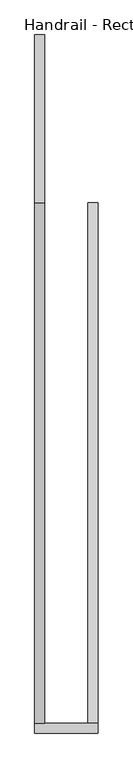
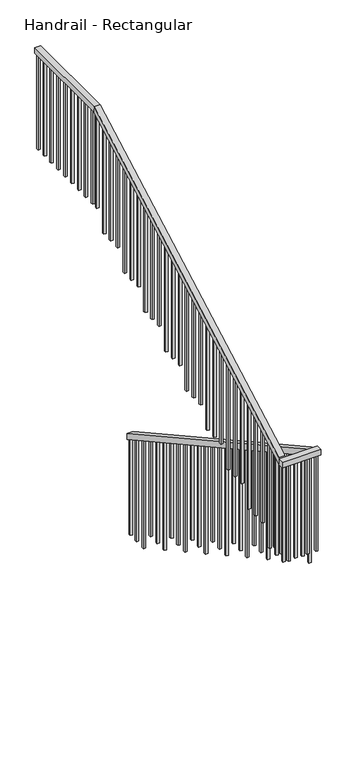
"""IFC4 building model written with IfcOpenShell, lengths in millimetres: railing geometry, Handrail - Rectangular."""

from ifc_helpers import new_model, si_unit, frame, origin, place, context, project, spatial, polyline, outline, extrude, faceted_brep, source, transform, mapped, element, save


def handrail_rectangular_766db315(model_context):
    return source(origin(), model_context, "Body", "SolidModel", [
        faceted_brep([(-74723.577375, 13792.2, 13481.05), (-74723.577375, 13792.2, 13430.25), (-74774.377375, 13792.2, 13430.25), (-74774.377375, 13792.2, 13481.05), (-74723.577375, 12915.9, 13481.05), (-74723.577375, 12929.0029811, 13430.25), (-74774.377375, 12929.0029811, 13430.25), (-74774.377375, 12915.9, 13481.05), (-74723.577375, 10198.1, 11979.1078947), (-74774.377375, 10198.1, 11979.1078947), (-74774.377375, 10198.1, 11921.0667736), (-74723.577375, 10198.1, 11921.0667736)], [[[0, 1, 2, 3]], [[1, 0, 4, 5]], [[2, 1, 5, 6]], [[3, 2, 6, 7]], [[0, 3, 7, 4]], [[8, 9, 10, 11]], [[5, 4, 8, 11]], [[6, 5, 11, 10]], [[7, 6, 10, 9]], [[4, 7, 9, 8]]]),
        faceted_brep([(-74774.377375, 10198.1, 11965.0710526), (-74774.377375, 10198.1, 11914.2710526), (-74774.377375, 10147.3, 11914.2710526), (-74774.377375, 10147.3, 11965.0710526), (-74444.177375, 10198.1, 11965.0710526), (-74444.177375, 10147.3, 11965.0710526), (-74444.177375, 10147.3, 11914.2710526), (-74444.177375, 10198.1, 11914.2710526)], [[[0, 1, 2, 3]], [[4, 5, 6, 7]], [[1, 0, 4, 7]], [[2, 1, 7, 6]], [[3, 2, 6, 5]], [[0, 3, 5, 4]]]),
        faceted_brep([(-74494.977375, 10198.1, 11951.0342105), (-74494.977375, 10198.1, 11892.9930894), (-74444.177375, 10198.1, 11892.9930894), (-74444.177375, 10198.1, 11951.0342105), (-74494.977375, 12915.9, 10449.0921053), (-74444.177375, 12915.9, 10449.0921053), (-74444.177375, 12915.9, 10391.0509841), (-74494.977375, 12915.9, 10391.0509841)], [[[0, 1, 2, 3]], [[4, 5, 6, 7]], [[1, 0, 4, 7]], [[2, 1, 7, 6]], [[3, 2, 6, 5]], [[0, 3, 5, 4]]]),
        extrude(outline(polyline([(12823.825, 10441.9345367), (12823.825, 9534.6921053), (12804.775, 9534.6921053), (12804.775, 10452.4621683), (12823.825, 10441.9345367)])), frame((-74479.102375, 0.0, 0.0), z_axis=(1.0, 0.0, 0.0), x_axis=(0.0, 1.0, 0.0)), (0.0, 0.0, 1.0), 19.05),
        extrude(outline(polyline([(12722.225, 10498.0819052), (12722.225, 9534.6921053), (12703.175, 9534.6921053), (12703.175, 10508.6095367), (12722.225, 10498.0819052)])), frame((-74479.102375, 0.0, 0.0), z_axis=(1.0, 0.0, 0.0), x_axis=(0.0, 1.0, 0.0)), (0.0, 0.0, 1.0), 19.05),
        extrude(outline(polyline([(12620.625, 10554.2292736), (12620.625, 9703.1342105), (12601.575, 9703.1342105), (12601.575, 10564.7569052), (12620.625, 10554.2292736)])), frame((-74479.102375, 0.0, 0.0), z_axis=(1.0, 0.0, 0.0), x_axis=(0.0, 1.0, 0.0)), (0.0, 0.0, 1.0), 19.05),
        extrude(outline(polyline([(12519.025, 10610.376642), (12519.025, 9703.1342105), (12499.975, 9703.1342105), (12499.975, 10620.9042736), (12519.025, 10610.376642)])), frame((-74479.102375, 0.0, 0.0), z_axis=(1.0, 0.0, 0.0), x_axis=(0.0, 1.0, 0.0)), (0.0, 0.0, 1.0), 19.05),
        extrude(outline(polyline([(12417.425, 10666.5240104), (12417.425, 9703.1342105), (12398.375, 9703.1342105), (12398.375, 10677.051642), (12417.425, 10666.5240104)])), frame((-74479.102375, 0.0, 0.0), z_axis=(1.0, 0.0, 0.0), x_axis=(0.0, 1.0, 0.0)), (0.0, 0.0, 1.0), 19.05),
        extrude(outline(polyline([(12315.825, 10722.6713788), (12315.825, 9871.5763158), (12296.775, 9871.5763158), (12296.775, 10733.1990104), (12315.825, 10722.6713788)])), frame((-74479.102375, 0.0, 0.0), z_axis=(1.0, 0.0, 0.0), x_axis=(0.0, 1.0, 0.0)), (0.0, 0.0, 1.0), 19.05),
        extrude(outline(polyline([(12214.225, 10778.8187473), (12214.225, 9871.5763158), (12195.175, 9871.5763158), (12195.175, 10789.3463788), (12214.225, 10778.8187473)])), frame((-74479.102375, 0.0, 0.0), z_axis=(1.0, 0.0, 0.0), x_axis=(0.0, 1.0, 0.0)), (0.0, 0.0, 1.0), 19.05),
        extrude(outline(polyline([(12112.625, 10834.9661157), (12112.625, 9871.5763158), (12093.575, 9871.5763158), (12093.575, 10845.4937473), (12112.625, 10834.9661157)])), frame((-74479.102375, 0.0, 0.0), z_axis=(1.0, 0.0, 0.0), x_axis=(0.0, 1.0, 0.0)), (0.0, 0.0, 1.0), 19.05),
        extrude(outline(polyline([(12011.025, 10891.1134841), (12011.025, 10040.0184211), (11991.975, 10040.0184211), (11991.975, 10901.6411157), (12011.025, 10891.1134841)])), frame((-74479.102375, 0.0, 0.0), z_axis=(1.0, 0.0, 0.0), x_axis=(0.0, 1.0, 0.0)), (0.0, 0.0, 1.0), 19.05),
        extrude(outline(polyline([(11909.425, 10947.2608525), (11909.425, 10040.0184211), (11890.375, 10040.0184211), (11890.375, 10957.7884841), (11909.425, 10947.2608525)])), frame((-74479.102375, 0.0, 0.0), z_axis=(1.0, 0.0, 0.0), x_axis=(0.0, 1.0, 0.0)), (0.0, 0.0, 1.0), 19.05),
        extrude(outline(polyline([(11807.825, 11003.4082209), (11807.825, 10040.0184211), (11788.775, 10040.0184211), (11788.775, 11013.9358525), (11807.825, 11003.4082209)])), frame((-74479.102375, 0.0, 0.0), z_axis=(1.0, 0.0, 0.0), x_axis=(0.0, 1.0, 0.0)), (0.0, 0.0, 1.0), 19.05),
        extrude(outline(polyline([(11706.225, 11059.5555894), (11706.225, 10208.4605263), (11687.175, 10208.4605263), (11687.175, 11070.0832209), (11706.225, 11059.5555894)])), frame((-74479.102375, 0.0, 0.0), z_axis=(1.0, 0.0, 0.0), x_axis=(0.0, 1.0, 0.0)), (0.0, 0.0, 1.0), 19.05),
        extrude(outline(polyline([(11604.625, 11115.7029578), (11604.625, 10208.4605263), (11585.575, 10208.4605263), (11585.575, 11126.2305894), (11604.625, 11115.7029578)])), frame((-74479.102375, 0.0, 0.0), z_axis=(1.0, 0.0, 0.0), x_axis=(0.0, 1.0, 0.0)), (0.0, 0.0, 1.0), 19.05),
        extrude(outline(polyline([(11503.025, 11171.8503262), (11503.025, 10208.4605263), (11483.975, 10208.4605263), (11483.975, 11182.3779578), (11503.025, 11171.8503262)])), frame((-74479.102375, 0.0, 0.0), z_axis=(1.0, 0.0, 0.0), x_axis=(0.0, 1.0, 0.0)), (0.0, 0.0, 1.0), 19.05),
        extrude(outline(polyline([(11401.425, 11227.9976946), (11401.425, 10376.9026316), (11382.375, 10376.9026316), (11382.375, 11238.5253262), (11401.425, 11227.9976946)])), frame((-74479.102375, 0.0, 0.0), z_axis=(1.0, 0.0, 0.0), x_axis=(0.0, 1.0, 0.0)), (0.0, 0.0, 1.0), 19.05),
        extrude(outline(polyline([(11299.825, 11284.1450631), (11299.825, 10376.9026316), (11280.775, 10376.9026316), (11280.775, 11294.6726946), (11299.825, 11284.1450631)])), frame((-74479.102375, 0.0, 0.0), z_axis=(1.0, 0.0, 0.0), x_axis=(0.0, 1.0, 0.0)), (0.0, 0.0, 1.0), 19.05),
        extrude(outline(polyline([(11198.225, 11340.2924315), (11198.225, 10376.9026316), (11179.175, 10376.9026316), (11179.175, 11350.8200631), (11198.225, 11340.2924315)])), frame((-74479.102375, 0.0, 0.0), z_axis=(1.0, 0.0, 0.0), x_axis=(0.0, 1.0, 0.0)), (0.0, 0.0, 1.0), 19.05),
        extrude(outline(polyline([(11096.625, 11396.4397999), (11096.625, 10545.3447368), (11077.575, 10545.3447368), (11077.575, 11406.9674315), (11096.625, 11396.4397999)])), frame((-74479.102375, 0.0, 0.0), z_axis=(1.0, 0.0, 0.0), x_axis=(0.0, 1.0, 0.0)), (0.0, 0.0, 1.0), 19.05),
        extrude(outline(polyline([(10995.025, 11452.5871683), (10995.025, 10545.3447368), (10975.975, 10545.3447368), (10975.975, 11463.1147999), (10995.025, 11452.5871683)])), frame((-74479.102375, 0.0, 0.0), z_axis=(1.0, 0.0, 0.0), x_axis=(0.0, 1.0, 0.0)), (0.0, 0.0, 1.0), 19.05),
        extrude(outline(polyline([(10893.425, 11508.7345367), (10893.425, 10545.3447368), (10874.375, 10545.3447368), (10874.375, 11519.2621683), (10893.425, 11508.7345367)])), frame((-74479.102375, 0.0, 0.0), z_axis=(1.0, 0.0, 0.0), x_axis=(0.0, 1.0, 0.0)), (0.0, 0.0, 1.0), 19.05),
        extrude(outline(polyline([(10791.825, 11564.8819052), (10791.825, 10713.7868421), (10772.775, 10713.7868421), (10772.775, 11575.4095367), (10791.825, 11564.8819052)])), frame((-74479.102375, 0.0, 0.0), z_axis=(1.0, 0.0, 0.0), x_axis=(0.0, 1.0, 0.0)), (0.0, 0.0, 1.0), 19.05),
        extrude(outline(polyline([(10690.225, 11621.0292736), (10690.225, 10713.7868421), (10671.175, 10713.7868421), (10671.175, 11631.5569052), (10690.225, 11621.0292736)])), frame((-74479.102375, 0.0, 0.0), z_axis=(1.0, 0.0, 0.0), x_axis=(0.0, 1.0, 0.0)), (0.0, 0.0, 1.0), 19.05),
        extrude(outline(polyline([(10588.625, 11677.176642), (10588.625, 10713.7868421), (10569.575, 10713.7868421), (10569.575, 11687.7042736), (10588.625, 11677.176642)])), frame((-74479.102375, 0.0, 0.0), z_axis=(1.0, 0.0, 0.0), x_axis=(0.0, 1.0, 0.0)), (0.0, 0.0, 1.0), 19.05),
        extrude(outline(polyline([(10487.025, 11733.3240104), (10487.025, 10882.2289474), (10467.975, 10882.2289474), (10467.975, 11743.851642), (10487.025, 11733.3240104)])), frame((-74479.102375, 0.0, 0.0), z_axis=(1.0, 0.0, 0.0), x_axis=(0.0, 1.0, 0.0)), (0.0, 0.0, 1.0), 19.05),
        extrude(outline(polyline([(10385.425, 11789.4713788), (10385.425, 10882.2289474), (10366.375, 10882.2289474), (10366.375, 11799.9990104), (10385.425, 11789.4713788)])), frame((-74479.102375, 0.0, 0.0), z_axis=(1.0, 0.0, 0.0), x_axis=(0.0, 1.0, 0.0)), (0.0, 0.0, 1.0), 19.05),
        extrude(outline(polyline([(10283.825, 11845.6187473), (10283.825, 10882.2289474), (10264.775, 10882.2289474), (10264.775, 11856.1463788), (10283.825, 11845.6187473)])), frame((-74479.102375, 0.0, 0.0), z_axis=(1.0, 0.0, 0.0), x_axis=(0.0, 1.0, 0.0)), (0.0, 0.0, 1.0), 19.05),
        extrude(outline(polyline([(-74555.302375, 10182.225), (-74536.252375, 10182.225), (-74536.252375, 10163.175), (-74555.302375, 10163.175), (-74555.302375, 10182.225)])), frame((0.0, 0.0, 11050.6710526), z_axis=(0.0, 0.0, 1.0), x_axis=(1.0, 0.0, 0.0)), (0.0, 0.0, 1.0), 863.6),
        extrude(outline(polyline([(-74656.902375, 10182.225), (-74637.852375, 10182.225), (-74637.852375, 10163.175), (-74656.902375, 10163.175), (-74656.902375, 10182.225)])), frame((0.0, 0.0, 11050.6710526), z_axis=(0.0, 0.0, 1.0), x_axis=(1.0, 0.0, 0.0)), (0.0, 0.0, 1.0), 863.6),
        extrude(outline(polyline([(10283.825, 11968.4411157), (10283.825, 11050.6710526), (10264.775, 11050.6710526), (10264.775, 11957.9134841), (10283.825, 11968.4411157)])), frame((-74758.502375, 0.0, 0.0), z_axis=(1.0, 0.0, 0.0), x_axis=(0.0, 1.0, 0.0)), (0.0, 0.0, 1.0), 19.05),
        extrude(outline(polyline([(10385.425, 12024.5884841), (10385.425, 11050.6710526), (10366.375, 11050.6710526), (10366.375, 12014.0608525), (10385.425, 12024.5884841)])), frame((-74758.502375, 0.0, 0.0), z_axis=(1.0, 0.0, 0.0), x_axis=(0.0, 1.0, 0.0)), (0.0, 0.0, 1.0), 19.05),
        extrude(outline(polyline([(10487.025, 12080.7358525), (10487.025, 11219.1131579), (10467.975, 11219.1131579), (10467.975, 12070.2082209), (10487.025, 12080.7358525)])), frame((-74758.502375, 0.0, 0.0), z_axis=(1.0, 0.0, 0.0), x_axis=(0.0, 1.0, 0.0)), (0.0, 0.0, 1.0), 19.05),
        extrude(outline(polyline([(10588.625, 12136.8832209), (10588.625, 11219.1131579), (10569.575, 11219.1131579), (10569.575, 12126.3555894), (10588.625, 12136.8832209)])), frame((-74758.502375, 0.0, 0.0), z_axis=(1.0, 0.0, 0.0), x_axis=(0.0, 1.0, 0.0)), (0.0, 0.0, 1.0), 19.05),
        extrude(outline(polyline([(10690.225, 12193.0305894), (10690.225, 11219.1131579), (10671.175, 11219.1131579), (10671.175, 12182.5029578), (10690.225, 12193.0305894)])), frame((-74758.502375, 0.0, 0.0), z_axis=(1.0, 0.0, 0.0), x_axis=(0.0, 1.0, 0.0)), (0.0, 0.0, 1.0), 19.05),
        extrude(outline(polyline([(10791.825, 12249.1779578), (10791.825, 11387.5552632), (10772.775, 11387.5552632), (10772.775, 12238.6503262), (10791.825, 12249.1779578)])), frame((-74758.502375, 0.0, 0.0), z_axis=(1.0, 0.0, 0.0), x_axis=(0.0, 1.0, 0.0)), (0.0, 0.0, 1.0), 19.05),
        extrude(outline(polyline([(10893.425, 12305.3253262), (10893.425, 11387.5552632), (10874.375, 11387.5552632), (10874.375, 12294.7976946), (10893.425, 12305.3253262)])), frame((-74758.502375, 0.0, 0.0), z_axis=(1.0, 0.0, 0.0), x_axis=(0.0, 1.0, 0.0)), (0.0, 0.0, 1.0), 19.05),
        extrude(outline(polyline([(10995.025, 12361.4726946), (10995.025, 11387.5552632), (10975.975, 11387.5552632), (10975.975, 12350.9450631), (10995.025, 12361.4726946)])), frame((-74758.502375, 0.0, 0.0), z_axis=(1.0, 0.0, 0.0), x_axis=(0.0, 1.0, 0.0)), (0.0, 0.0, 1.0), 19.05),
        extrude(outline(polyline([(11096.625, 12417.6200631), (11096.625, 11555.9973684), (11077.575, 11555.9973684), (11077.575, 12407.0924315), (11096.625, 12417.6200631)])), frame((-74758.502375, 0.0, 0.0), z_axis=(1.0, 0.0, 0.0), x_axis=(0.0, 1.0, 0.0)), (0.0, 0.0, 1.0), 19.05),
        extrude(outline(polyline([(11198.225, 12473.7674315), (11198.225, 11555.9973684), (11179.175, 11555.9973684), (11179.175, 12463.2397999), (11198.225, 12473.7674315)])), frame((-74758.502375, 0.0, 0.0), z_axis=(1.0, 0.0, 0.0), x_axis=(0.0, 1.0, 0.0)), (0.0, 0.0, 1.0), 19.05),
        extrude(outline(polyline([(11299.825, 12529.9147999), (11299.825, 11555.9973684), (11280.775, 11555.9973684), (11280.775, 12519.3871683), (11299.825, 12529.9147999)])), frame((-74758.502375, 0.0, 0.0), z_axis=(1.0, 0.0, 0.0), x_axis=(0.0, 1.0, 0.0)), (0.0, 0.0, 1.0), 19.05),
        extrude(outline(polyline([(11401.425, 12586.0621683), (11401.425, 11724.4394737), (11382.375, 11724.4394737), (11382.375, 12575.5345367), (11401.425, 12586.0621683)])), frame((-74758.502375, 0.0, 0.0), z_axis=(1.0, 0.0, 0.0), x_axis=(0.0, 1.0, 0.0)), (0.0, 0.0, 1.0), 19.05),
        extrude(outline(polyline([(11503.025, 12642.2095367), (11503.025, 11724.4394737), (11483.975, 11724.4394737), (11483.975, 12631.6819052), (11503.025, 12642.2095367)])), frame((-74758.502375, 0.0, 0.0), z_axis=(1.0, 0.0, 0.0), x_axis=(0.0, 1.0, 0.0)), (0.0, 0.0, 1.0), 19.05),
        extrude(outline(polyline([(11604.625, 12698.3569052), (11604.625, 11724.4394737), (11585.575, 11724.4394737), (11585.575, 12687.8292736), (11604.625, 12698.3569052)])), frame((-74758.502375, 0.0, 0.0), z_axis=(1.0, 0.0, 0.0), x_axis=(0.0, 1.0, 0.0)), (0.0, 0.0, 1.0), 19.05),
        extrude(outline(polyline([(11706.225, 12754.5042736), (11706.225, 11892.8815789), (11687.175, 11892.8815789), (11687.175, 12743.976642), (11706.225, 12754.5042736)])), frame((-74758.502375, 0.0, 0.0), z_axis=(1.0, 0.0, 0.0), x_axis=(0.0, 1.0, 0.0)), (0.0, 0.0, 1.0), 19.05),
        extrude(outline(polyline([(11807.825, 12810.651642), (11807.825, 11892.8815789), (11788.775, 11892.8815789), (11788.775, 12800.1240104), (11807.825, 12810.651642)])), frame((-74758.502375, 0.0, 0.0), z_axis=(1.0, 0.0, 0.0), x_axis=(0.0, 1.0, 0.0)), (0.0, 0.0, 1.0), 19.05),
        extrude(outline(polyline([(11909.425, 12866.7990104), (11909.425, 11892.8815789), (11890.375, 11892.8815789), (11890.375, 12856.2713788), (11909.425, 12866.7990104)])), frame((-74758.502375, 0.0, 0.0), z_axis=(1.0, 0.0, 0.0), x_axis=(0.0, 1.0, 0.0)), (0.0, 0.0, 1.0), 19.05),
        extrude(outline(polyline([(12011.025, 12922.9463788), (12011.025, 12061.3236842), (11991.975, 12061.3236842), (11991.975, 12912.4187473), (12011.025, 12922.9463788)])), frame((-74758.502375, 0.0, 0.0), z_axis=(1.0, 0.0, 0.0), x_axis=(0.0, 1.0, 0.0)), (0.0, 0.0, 1.0), 19.05),
        extrude(outline(polyline([(12112.625, 12979.0937473), (12112.625, 12061.3236842), (12093.575, 12061.3236842), (12093.575, 12968.5661157), (12112.625, 12979.0937473)])), frame((-74758.502375, 0.0, 0.0), z_axis=(1.0, 0.0, 0.0), x_axis=(0.0, 1.0, 0.0)), (0.0, 0.0, 1.0), 19.05),
        extrude(outline(polyline([(12214.225, 13035.2411157), (12214.225, 12061.3236842), (12195.175, 12061.3236842), (12195.175, 13024.7134841), (12214.225, 13035.2411157)])), frame((-74758.502375, 0.0, 0.0), z_axis=(1.0, 0.0, 0.0), x_axis=(0.0, 1.0, 0.0)), (0.0, 0.0, 1.0), 19.05),
        extrude(outline(polyline([(12315.825, 13091.3884841), (12315.825, 12229.7657895), (12296.775, 12229.7657895), (12296.775, 13080.8608525), (12315.825, 13091.3884841)])), frame((-74758.502375, 0.0, 0.0), z_axis=(1.0, 0.0, 0.0), x_axis=(0.0, 1.0, 0.0)), (0.0, 0.0, 1.0), 19.05),
        extrude(outline(polyline([(12417.425, 13147.5358525), (12417.425, 12229.7657895), (12398.375, 12229.7657895), (12398.375, 13137.0082209), (12417.425, 13147.5358525)])), frame((-74758.502375, 0.0, 0.0), z_axis=(1.0, 0.0, 0.0), x_axis=(0.0, 1.0, 0.0)), (0.0, 0.0, 1.0), 19.05),
        extrude(outline(polyline([(12519.025, 13203.6832209), (12519.025, 12229.7657895), (12499.975, 12229.7657895), (12499.975, 13193.1555894), (12519.025, 13203.6832209)])), frame((-74758.502375, 0.0, 0.0), z_axis=(1.0, 0.0, 0.0), x_axis=(0.0, 1.0, 0.0)), (0.0, 0.0, 1.0), 19.05),
        extrude(outline(polyline([(12620.625, 13259.8305894), (12620.625, 12398.2078947), (12601.575, 12398.2078947), (12601.575, 13249.3029578), (12620.625, 13259.8305894)])), frame((-74758.502375, 0.0, 0.0), z_axis=(1.0, 0.0, 0.0), x_axis=(0.0, 1.0, 0.0)), (0.0, 0.0, 1.0), 19.05),
        extrude(outline(polyline([(12722.225, 13315.9779578), (12722.225, 12398.2078947), (12703.175, 12398.2078947), (12703.175, 13305.4503262), (12722.225, 13315.9779578)])), frame((-74758.502375, 0.0, 0.0), z_axis=(1.0, 0.0, 0.0), x_axis=(0.0, 1.0, 0.0)), (0.0, 0.0, 1.0), 19.05),
        extrude(outline(polyline([(12823.825, 13372.1253262), (12823.825, 12398.2078947), (12804.775, 12398.2078947), (12804.775, 13361.5976946), (12823.825, 13372.1253262)])), frame((-74758.502375, 0.0, 0.0), z_axis=(1.0, 0.0, 0.0), x_axis=(0.0, 1.0, 0.0)), (0.0, 0.0, 1.0), 19.05),
        extrude(outline(polyline([(-74739.452375, 12988.925), (-74739.452375, 12969.875), (-74758.502375, 12969.875), (-74758.502375, 12988.925), (-74739.452375, 12988.925)])), frame((0.0, 0.0, 12566.65), z_axis=(0.0, 0.0, 1.0), x_axis=(1.0, 0.0, 0.0)), (0.0, 0.0, 1.0), 863.6),
        extrude(outline(polyline([(-74739.452375, 13090.525), (-74739.452375, 13071.475), (-74758.502375, 13071.475), (-74758.502375, 13090.525), (-74739.452375, 13090.525)])), frame((0.0, 0.0, 12566.65), z_axis=(0.0, 0.0, 1.0), x_axis=(1.0, 0.0, 0.0)), (0.0, 0.0, 1.0), 863.6),
        extrude(outline(polyline([(-74739.452375, 13192.125), (-74739.452375, 13173.075), (-74758.502375, 13173.075), (-74758.502375, 13192.125), (-74739.452375, 13192.125)])), frame((0.0, 0.0, 12566.65), z_axis=(0.0, 0.0, 1.0), x_axis=(1.0, 0.0, 0.0)), (0.0, 0.0, 1.0), 863.6),
        extrude(outline(polyline([(-74739.452375, 13293.725), (-74739.452375, 13274.675), (-74758.502375, 13274.675), (-74758.502375, 13293.725), (-74739.452375, 13293.725)])), frame((0.0, 0.0, 12566.65), z_axis=(0.0, 0.0, 1.0), x_axis=(1.0, 0.0, 0.0)), (0.0, 0.0, 1.0), 863.6),
        extrude(outline(polyline([(-74739.452375, 13395.325), (-74739.452375, 13376.275), (-74758.502375, 13376.275), (-74758.502375, 13395.325), (-74739.452375, 13395.325)])), frame((0.0, 0.0, 12566.65), z_axis=(0.0, 0.0, 1.0), x_axis=(1.0, 0.0, 0.0)), (0.0, 0.0, 1.0), 863.6),
        extrude(outline(polyline([(-74739.452375, 13496.925), (-74739.452375, 13477.875), (-74758.502375, 13477.875), (-74758.502375, 13496.925), (-74739.452375, 13496.925)])), frame((0.0, 0.0, 12566.65), z_axis=(0.0, 0.0, 1.0), x_axis=(1.0, 0.0, 0.0)), (0.0, 0.0, 1.0), 863.6),
        extrude(outline(polyline([(-74739.452375, 13598.525), (-74739.452375, 13579.475), (-74758.502375, 13579.475), (-74758.502375, 13598.525), (-74739.452375, 13598.525)])), frame((0.0, 0.0, 12566.65), z_axis=(0.0, 0.0, 1.0), x_axis=(1.0, 0.0, 0.0)), (0.0, 0.0, 1.0), 863.6),
        extrude(outline(polyline([(-74739.452375, 13700.125), (-74739.452375, 13681.075), (-74758.502375, 13681.075), (-74758.502375, 13700.125), (-74739.452375, 13700.125)])), frame((0.0, 0.0, 12566.65), z_axis=(0.0, 0.0, 1.0), x_axis=(1.0, 0.0, 0.0)), (0.0, 0.0, 1.0), 863.6),
        extrude(outline(polyline([(-74479.102375, 10182.225), (-74460.052375, 10182.225), (-74460.052375, 10163.175), (-74479.102375, 10163.175), (-74479.102375, 10182.225)])), frame((0.0, 0.0, 11050.6710526), z_axis=(0.0, 0.0, 1.0), x_axis=(1.0, 0.0, 0.0)), (0.0, 0.0, 1.0), 863.6),
        extrude(outline(polyline([(10182.225, 11912.2937473), (10182.225, 11050.6710526), (10163.175, 11050.6710526), (10163.175, 11901.7661157), (10182.225, 11912.2937473)])), frame((-74758.502375, 0.0, 0.0), z_axis=(1.0, 0.0, 0.0), x_axis=(0.0, 1.0, 0.0)), (0.0, 0.0, 1.0), 19.05),
        extrude(outline(polyline([(-74739.452375, 12925.425), (-74739.452375, 12906.375), (-74758.502375, 12906.375), (-74758.502375, 12925.425), (-74739.452375, 12925.425)])), frame((0.0, 0.0, 12566.65), z_axis=(0.0, 0.0, 1.0), x_axis=(1.0, 0.0, 0.0)), (0.0, 0.0, 1.0), 863.6),
        extrude(outline(polyline([(12915.9, 10391.0509841), (12915.9, 9534.6921053), (12896.85, 9534.6921053), (12896.85, 10401.5786157), (12915.9, 10391.0509841)])), frame((-74479.102375, 0.0, 0.0), z_axis=(1.0, 0.0, 0.0), x_axis=(0.0, 1.0, 0.0)), (0.0, 0.0, 1.0), 19.05),
        extrude(outline(polyline([(-74739.452375, 13792.2), (-74739.452375, 13773.15), (-74758.502375, 13773.15), (-74758.502375, 13792.2), (-74739.452375, 13792.2)])), frame((0.0, 0.0, 12566.65), z_axis=(0.0, 0.0, 1.0), x_axis=(1.0, 0.0, 0.0)), (0.0, 0.0, 1.0), 863.6),
    ])


if __name__ == "__main__":
    model = new_model("IFC4")
    model_context = context("Model", 3, world=origin())
    ifc_project = project(units=[si_unit("LENGTHUNIT", "METRE", prefix="MILLI")], contexts=[model_context])
    site = spatial("IfcSite", under=ifc_project)
    building = spatial("IfcBuilding", under=site)
    placement = place(None, origin())
    handrail_rectangular_shape = handrail_rectangular_766db315(model_context)
    element("IfcRailing", 1, ObjectType="Handrail - Rectangular", at=placement, inside=building, context=model_context, shape_type="MappedRepresentation", body=[
        mapped(handrail_rectangular_shape, transform((0.0, 0.0, 0.0), x_axis=(1.0, 0.0, 0.0), y_axis=(0.0, 1.0, 0.0), z_axis=(0.0, 0.0, 1.0))),
    ])
    save(model, "model.ifc")
